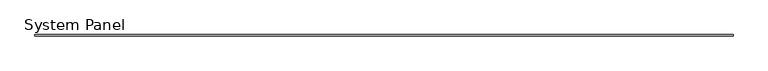
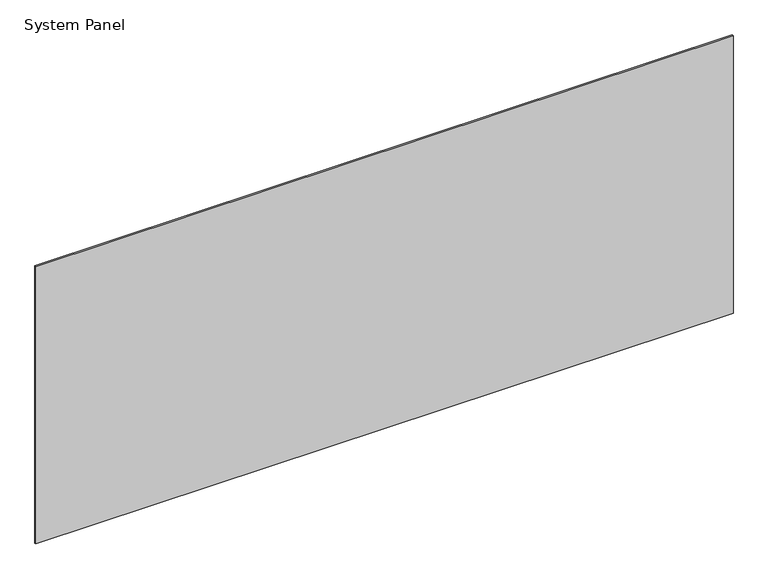
"""IFC4 building model written with IfcOpenShell, lengths in millimetres: plate geometry, System Panel : 로이복층유리_16."""

from ifc_helpers import new_model, si_unit, origin, origin_with_axes, place, context, project, spatial, polyline, outline, extrude, source, transform, mapped, element, save


def system_panel_25601cef(model_context):
    return source(origin(), model_context, "Body", "SweptSolid", [
        extrude(outline(polyline([(3580.0000001, -8.0), (-3580.0000001, -8.0), (-3580.0000001, 8.0), (3580.0000001, 8.0), (3580.0000001, -8.0)])), origin_with_axes(), (0.0, 0.0, 1.0), 3010.0),
    ])


if __name__ == "__main__":
    model = new_model("IFC4")
    model_context = context("Model", 3, world=origin())
    ifc_project = project(units=[si_unit("LENGTHUNIT", "METRE", prefix="MILLI")], contexts=[model_context])
    site = spatial("IfcSite", under=ifc_project)
    building = spatial("IfcBuilding", under=site)
    placement = place(None, origin())
    system_panel_shape = system_panel_25601cef(model_context)
    element("IfcPlate", 1, ObjectType="System Panel : 로이복층유리_16", at=placement, inside=building, context=model_context, shape_type="MappedRepresentation", body=[
        mapped(system_panel_shape, transform((0.0, 0.0, 0.0), x_axis=(1.0, 0.0, 0.0), y_axis=(0.0, 1.0, 0.0), z_axis=(0.0, 0.0, 1.0))),
    ])
    save(model, "model.ifc")

# Revit data of these elements
# Element 1 (IfcPlate, "System Panel : 로이복층유리_16")
#   Materials on its faces: "00_Glass_Glass"
# Materials
#   "00_Glass_Glass": class "Glass", colour RGB 218 227 224, transparency 0.85, Description = "Glass", Cost = 0, Image = none
